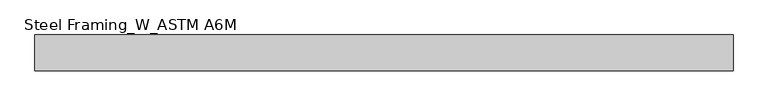
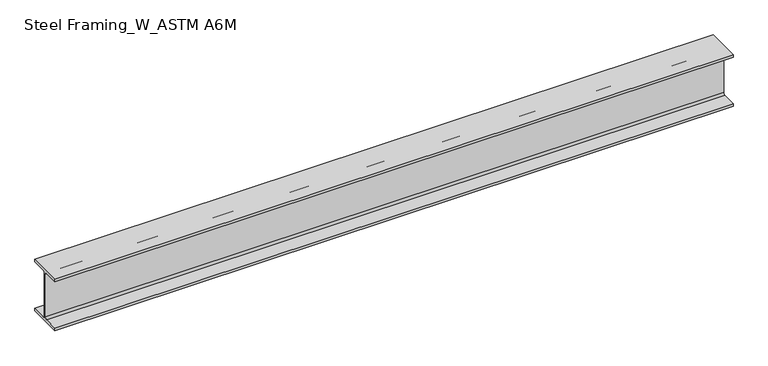
"""IFC4 building model written with IfcOpenShell, lengths in millimetres: beam geometry, Steel Framing_W_ASTM A6M : H_SB_AR_S02_W200x31.3_B6."""

import ifcopenshell
import ifcopenshell.guid

model = None  # the IFC model being written
_history = None  # IfcOwnerHistory: only IFC2X3 demands one
_inside = {}  # id of a spatial element -> (the spatial element, [elements in it])
_under = {}  # id of a project, library or spatial element -> (it, [spatial elements below it])
_declared = {}  # id of a project -> (the project, [libraries it declares])
_typed = {}  # id of a type object -> (the type object, [elements of that type])
_made_of = {}  # id of a material, layer set ... -> (it, [elements and type objects made of it])


def new_model(schema):
    """Start an empty IFC model of exactly this schema.

    Asked for "IFC4X3", IfcOpenShell would pick the latest addendum, in which some entities
    have other attributes; the version numbers below select the first issue.
    IFC2X3 requires an IfcOwnerHistory on every rooted entity: one is made here for all.
    """
    global model, _history
    if schema == "IFC4X3":
        model = ifcopenshell.file(schema_version=(4, 3, 0, 0))
    else:
        model = ifcopenshell.file(schema=schema)
    _inside.clear()
    _under.clear()
    _declared.clear()
    _typed.clear()
    _made_of.clear()
    _history = None
    if model.schema == "IFC2X3":
        org = make("IfcOrganization", Name="unknown")
        user = make(
            "IfcPersonAndOrganization",
            ThePerson=make("IfcPerson", FamilyName="unknown"),
            TheOrganization=org,
        )
        app = make(
            "IfcApplication",
            ApplicationDeveloper=org,
            Version="unknown",
            ApplicationFullName="unknown",
            ApplicationIdentifier="unknown",
        )
        _history = make(
            "IfcOwnerHistory",
            OwningUser=user,
            OwningApplication=app,
            ChangeAction="ADDED",
            CreationDate=0,
        )
    return model


def make(cls, **values):
    """One entity of the class cls with the attributes given. An attribute that is None is left unset."""
    return model.create_entity(
        cls, **{name: value for name, value in values.items() if value is not None}
    )


def rooted(cls, **values):
    """An entity with a GlobalId (a new one), such as an element, a storey or a relation."""
    return make(cls, GlobalId=ifcopenshell.guid.new(), OwnerHistory=_history, **values)


def si_unit(unit_type, name, prefix=None):
    """IfcSIUnit, for example si_unit("LENGTHUNIT", "METRE", prefix="MILLI")."""
    return make("IfcSIUnit", UnitType=unit_type, Prefix=prefix, Name=name)


def assignment(units):
    """IfcUnitAssignment: the units of a project."""
    return None if units is None else make("IfcUnitAssignment", Units=units)


def point(xyz):
    """IfcCartesianPoint."""
    return None if xyz is None else make("IfcCartesianPoint", Coordinates=xyz)


def direction(xyz):
    """IfcDirection."""
    return None if xyz is None else make("IfcDirection", DirectionRatios=xyz)


def frame(location, z_axis=None, x_axis=None):
    """IfcAxis2Placement3D, a coordinate frame: its origin and axes. An axis left out is left unset."""
    return make(
        "IfcAxis2Placement3D",
        Location=point(location),
        Axis=direction(z_axis),
        RefDirection=direction(x_axis),
    )


def frame_2d(location, x_axis=None):
    """IfcAxis2Placement2D, a coordinate frame in the plane: its origin and x axis."""
    return make(
        "IfcAxis2Placement2D", Location=point(location), RefDirection=direction(x_axis)
    )


def origin():
    """The frame at (0, 0, 0) with its axes left unset."""
    return frame((0.0, 0.0, 0.0))


def place(relative_to, where):
    """IfcLocalPlacement: puts the frame where relative to a parent placement (None: the world)."""
    return make(
        "IfcLocalPlacement", PlacementRelTo=relative_to, RelativePlacement=where
    )


def context(
    kind, dimensions, precision=None, world=None, true_north=None, identifier=None
):
    """IfcGeometricRepresentationContext, for example the 3D "Model" context."""
    return make(
        "IfcGeometricRepresentationContext",
        ContextIdentifier=identifier,
        ContextType=kind,
        CoordinateSpaceDimension=dimensions,
        Precision=precision,
        WorldCoordinateSystem=world,
        TrueNorth=true_north,
    )


def project(units=None, contexts=None):
    """IfcProject with its units and contexts."""
    return rooted(
        "IfcProject",
        Name="project",
        RepresentationContexts=contexts,
        UnitsInContext=assignment(units),
    )


def spatial(cls, under=None, at=None, **own):
    """A site, building, storey or space (cls), placed at a placement, below another one or the project."""
    s = rooted(cls, ObjectPlacement=at, **own)
    if under is not None:
        _under.setdefault(under.id(), (under, []))[1].append(s)
    return s


def polyline(points):
    """IfcPolyline through the points."""
    return make("IfcPolyline", Points=[point(p) for p in points])


def circle_curve(where, radius):
    """IfcCircle in the frame where."""
    return make("IfcCircle", Position=where, Radius=radius)


def trimmed(basis, trim1, trim2, sense, master):
    """IfcTrimmedCurve: the piece of a basis curve between two trims."""
    return make(
        "IfcTrimmedCurve",
        BasisCurve=basis,
        Trim1=trim1,
        Trim2=trim2,
        SenseAgreement=sense,
        MasterRepresentation=master,
    )


def segment(curve, same_sense, transition):
    """IfcCompositeCurveSegment."""
    return make(
        "IfcCompositeCurveSegment",
        Transition=transition,
        SameSense=same_sense,
        ParentCurve=curve,
    )


def composite_curve(segments, self_intersect=None):
    """IfcCompositeCurve: segments joined end to end."""
    return make("IfcCompositeCurve", Segments=segments, SelfIntersect=self_intersect)


def outline(outer, holes=None, kind="AREA"):
    """IfcArbitraryClosedProfileDef: a profile drawn as a closed curve; with holes, ...WithVoids."""
    if holes is None:
        return make("IfcArbitraryClosedProfileDef", ProfileType=kind, OuterCurve=outer)
    return make(
        "IfcArbitraryProfileDefWithVoids",
        ProfileType=kind,
        OuterCurve=outer,
        InnerCurves=holes,
    )


def extrude(swept, where, along, depth):
    """IfcExtrudedAreaSolid: the profile swept, set in the frame where, extruded along a direction by depth."""
    return make(
        "IfcExtrudedAreaSolid",
        SweptArea=swept,
        Position=where,
        ExtrudedDirection=direction(along),
        Depth=depth,
    )


def shape(context_of_items, identifier, shape_type, items):
    """IfcShapeRepresentation: the items that make up one representation, for example the "Body"."""
    return make(
        "IfcShapeRepresentation",
        ContextOfItems=context_of_items,
        RepresentationIdentifier=identifier,
        RepresentationType=shape_type,
        Items=items,
    )


def source(mapping_origin, context_of_items, identifier, shape_type, items):
    """IfcRepresentationMap: a shape defined once, which mapped items show again and again."""
    return make(
        "IfcRepresentationMap",
        MappingOrigin=mapping_origin,
        MappedRepresentation=shape(context_of_items, identifier, shape_type, items),
    )


def transform(
    local_origin,
    x_axis=None,
    y_axis=None,
    z_axis=None,
    scale=None,
    scale2=None,
    scale3=None,
    uniform=True,
):
    """IfcCartesianTransformationOperator3D, or its non-uniform kind. x_axis, y_axis, z_axis: its Axis1, 2, 3."""
    if uniform:
        return make(
            "IfcCartesianTransformationOperator3D",
            Axis1=direction(x_axis),
            Axis2=direction(y_axis),
            LocalOrigin=point(local_origin),
            Scale=scale,
            Axis3=direction(z_axis),
        )
    return make(
        "IfcCartesianTransformationOperator3DnonUniform",
        Axis1=direction(x_axis),
        Axis2=direction(y_axis),
        LocalOrigin=point(local_origin),
        Scale=scale,
        Axis3=direction(z_axis),
        Scale2=scale2,
        Scale3=scale3,
    )


def mapped(mapping_source, mapping_target):
    """IfcMappedItem: shows the shape of a source again, moved by a transform."""
    return make(
        "IfcMappedItem", MappingSource=mapping_source, MappingTarget=mapping_target
    )


def made_of(thing, what):
    """Note that an element or type object is made of a material, layer set ...; save() writes the relation."""
    if what is not None:
        _made_of.setdefault(what.id(), (what, []))[1].append(thing)
    return thing


def element(
    cls,
    number,
    at=None,
    inside=None,
    cuts=None,
    type_object=None,
    material=None,
    context=None,
    identifier="Body",
    shape_type=None,
    held_by="IfcProductDefinitionShape",
    body=None,
    shapes=None,
    **own,
):
    """One element of the class cls, such as IfcWall. Its Tag is "e" and its number.

    at: its placement. inside: the storey or other place that contains it. cuts: it is an
    opening in that element (IfcRelVoidsElement). A single representation is given by context,
    identifier, shape_type and body (its items); several are given by shapes. held_by: the class
    of the entity that holds the representations. save() writes the other relations.
    """
    e = rooted(cls, Tag="e%d" % number, ObjectPlacement=at, **own)
    if body is not None:
        shapes = [shape(context, identifier, shape_type, body)]
    if shapes is not None:
        e.Representation = make(held_by, Representations=shapes)
    if inside is not None:
        _inside.setdefault(inside.id(), (inside, []))[1].append(e)
    if cuts is not None:
        rooted(
            "IfcRelVoidsElement", RelatingBuildingElement=cuts, RelatedOpeningElement=e
        )
    if type_object is not None:
        _typed.setdefault(type_object.id(), (type_object, []))[1].append(e)
    return made_of(e, material)


def aggregate(whole, parts):
    """IfcRelAggregates: a whole, such as a stair, and the parts it consists of."""
    return rooted("IfcRelAggregates", RelatingObject=whole, RelatedObjects=parts)


def save(model, path):
    """Write the relations noted so far, then the file.

    IfcRelAggregates (storeys below a building ...), IfcRelContainedInSpatialStructure (elements
    in a storey), IfcRelDefinesByType, IfcRelAssociatesMaterial and IfcRelDeclares: one each for
    every whole, place, type object, material and project.
    """
    for whole, parts in _under.values():
        aggregate(whole, parts)
    for where, things in _inside.values():
        rooted(
            "IfcRelContainedInSpatialStructure",
            RelatedElements=things,
            RelatingStructure=where,
        )
    for kind, things in _typed.values():
        rooted("IfcRelDefinesByType", RelatedObjects=things, RelatingType=kind)
    for what, things in _made_of.values():
        rooted("IfcRelAssociatesMaterial", RelatedObjects=things, RelatingMaterial=what)
    for by, libraries in _declared.values():
        rooted("IfcRelDeclares", RelatingContext=by, RelatedDefinitions=libraries)
    model.write(path)


def steel_framing_w_astm_a6m_04ed26ec(model_context):
    return source(origin(), model_context, "Body", "SweptSolid", [
        extrude(outline(composite_curve([segment(polyline([(67.0, -94.8), (67.0, -105.0), (-67.0, -105.0), (-67.0, -94.8), (-10.775, -94.8)]), True, "CONTINUOUS"), segment(trimmed(circle_curve(frame_2d((-10.775, -87.2)), 7.6), [point((-10.775, -94.8))], [point((-3.175, -87.2))], True, "CARTESIAN"), True, "CONTINUOUS"), segment(polyline([(-3.175, -87.2), (-3.175, 87.2)]), True, "CONTINUOUS"), segment(trimmed(circle_curve(frame_2d((-10.775, 87.2)), 7.6), [point((-3.175, 87.2))], [point((-10.775, 94.8))], True, "CARTESIAN"), True, "CONTINUOUS"), segment(polyline([(-10.775, 94.8), (-67.0, 94.8), (-67.0, 105.0), (67.0, 105.0), (67.0, 94.8), (10.775, 94.8)]), True, "CONTINUOUS"), segment(trimmed(circle_curve(frame_2d((10.775, 87.2)), 7.6), [point((10.775, 94.8))], [point((3.175, 87.2))], True, "CARTESIAN"), True, "CONTINUOUS"), segment(polyline([(3.175, 87.2), (3.175, -87.2)]), True, "CONTINUOUS"), segment(trimmed(circle_curve(frame_2d((10.775, -87.2)), 7.6), [point((3.175, -87.2))], [point((10.775, -94.8))], True, "CARTESIAN"), True, "CONTINUOUS"), segment(polyline([(10.775, -94.8), (67.0, -94.8)]), True, "CONTINUOUS")], self_intersect=False)), frame((-1346.3, 0.0, 0.0), z_axis=(1.0, 0.0, 0.0), x_axis=(0.0, 1.0, 0.0)), (0.0, 0.0, 1.0), 2620.8),
    ])


if __name__ == "__main__":
    model = new_model("IFC4")
    model_context = context("Model", 3, world=origin())
    ifc_project = project(units=[si_unit("LENGTHUNIT", "METRE", prefix="MILLI")], contexts=[model_context])
    site = spatial("IfcSite", under=ifc_project)
    building = spatial("IfcBuilding", under=site)
    placement = place(None, origin())
    steel_framing_w_astm_a6m_shape = steel_framing_w_astm_a6m_04ed26ec(model_context)
    element("IfcBeam", 1, ObjectType="Steel Framing_W_ASTM A6M : H_SB_AR_S02_W200x31.3_B6", at=placement, inside=building, context=model_context, shape_type="MappedRepresentation", body=[
        mapped(steel_framing_w_astm_a6m_shape, transform((0.0, 0.0, 0.0), x_axis=(1.0, 0.0, 0.0), y_axis=(0.0, 1.0, 0.0), z_axis=(0.0, 0.0, 1.0))),
    ])
    save(model, "model.ifc")

# Revit data of these elements
# Type "Steel Framing_W_ASTM A6M : H_SB_AR_S02_W200x31.3_B6"
#   Type Mark = "B6"
#   Section Name Key = "W8x21"
#   Width = 13.4 cm
#   Web Thickness = 0.635 cm
#   Web Fillet = 0.76 cm
#   Warping Constant = 40800.0 cm⁶
#   Torsional Moment of Inertia = 11.70 cm⁴
#   Section Area = 39.7 cm²
#   Plastic Modulus weak axis = 93.2 cm³
#   Plastic Modulus strong axis = 334.0 cm³
#   Perimeter = 0.93 m²/m
#   Nominal Weight = 31.30 kgf/m
#   Moment of Inertia weak axis = 407.00 cm⁴
#   Moment of Inertia strong axis = 3130.00 cm⁴
#   Height = 21.0 cm
#   Flange Thickness = 1.02 cm
#   Elastic Modulus weak axis = 60.8 cm³
#   Elastic Modulus strong axis = 298.0 cm³
#   Centroid Vertical = 10.5 cm
#   Centroid Horizontal = 6.7 cm
#   Length [instance default] = 1500 mm
#   Structural Material [instance default] = Steel, 45-345
#   Bolt Spacing = 0
#   Assembly Code = ""
# Element 1 (IfcBeam, "Steel Framing_W_ASTM A6M : H_SB_AR_S02_W200x31.3_B6")
#   Materials on its faces: "Steel, 45-345"
# Materials
#   "Steel, 45-345": class "Metal", colour RGB 189 187 185, transparency 0, Description = "Steel 345 MPa", Cost = 0
